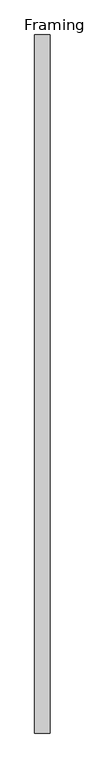
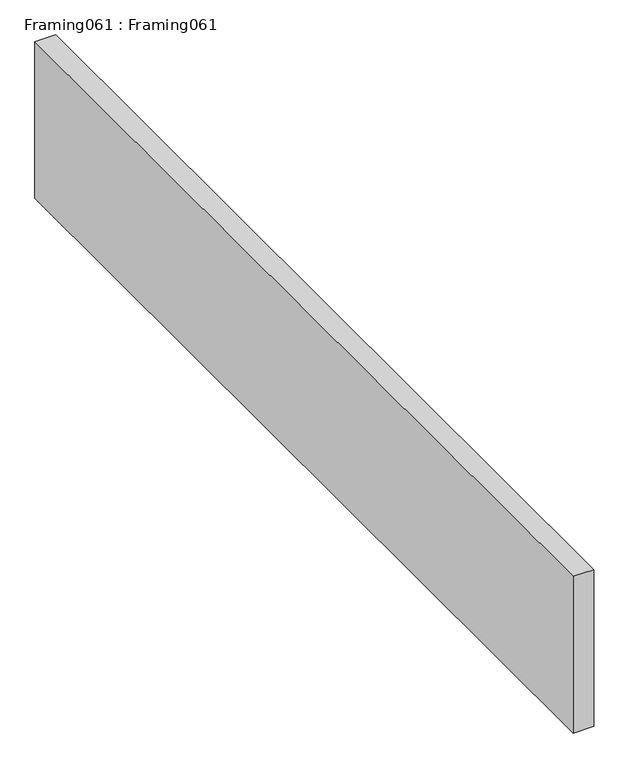
"""IFC4 building model written with IfcOpenShell, lengths in millimetres: proxy geometry, Framing061 : Framing061."""

from ifc_helpers import new_model, si_unit, frame, origin, place, context, project, spatial, polyline, outline, extrude, source, transform, mapped, element, save


def framing061_framing061_db29d32c(model_context):
    return source(origin(), model_context, "Body", "SweptSolid", [
        extrude(outline(polyline([(-1345.9885697, -1052.8906574), (-1390.4385697, -1052.8906574), (-1390.4385697, 947.1093426), (-1345.9885697, 947.1093426), (-1345.9885697, -1052.8906574)])), frame((0.0, 0.0, 42134.105552), z_axis=(0.0, 0.0, 1.0), x_axis=(1.0, 0.0, 0.0)), (0.0, 0.0, 1.0), 355.2981173),
    ])


if __name__ == "__main__":
    model = new_model("IFC4")
    model_context = context("Model", 3, world=origin())
    ifc_project = project(units=[si_unit("LENGTHUNIT", "METRE", prefix="MILLI")], contexts=[model_context])
    site = spatial("IfcSite", under=ifc_project)
    building = spatial("IfcBuilding", under=site)
    placement = place(None, origin())
    framing061_framing061_shape = framing061_framing061_db29d32c(model_context)
    element("IfcBuildingElementProxy", 1, Name="Framing061 : Framing061", ObjectType="Framing061 : Framing061", at=placement, inside=building, context=model_context, shape_type="MappedRepresentation", body=[
        mapped(framing061_framing061_shape, transform((0.0, 0.0, 0.0), x_axis=(1.0, 0.0, 0.0), y_axis=(0.0, 1.0, 0.0), z_axis=(0.0, 0.0, 1.0))),
    ])
    save(model, "model.ifc")

# Revit data of these elements
# Type "Framing061 : Framing061"
#   NameOverride = "Framing061"
# Element 1 (IfcBuildingElementProxy, "Framing061 : Framing061")
#   Materials on its faces: "WOOD FRAMING (SEE STRUCT DWGS)"
# Materials
#   "WOOD FRAMING (SEE STRUCT DWGS)": class "Unassigned", colour RGB 224 188 168, transparency 0, Cost = 0
